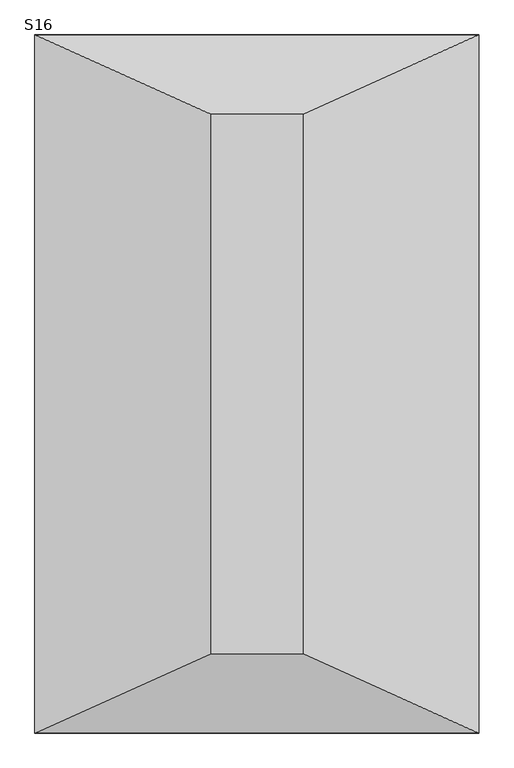
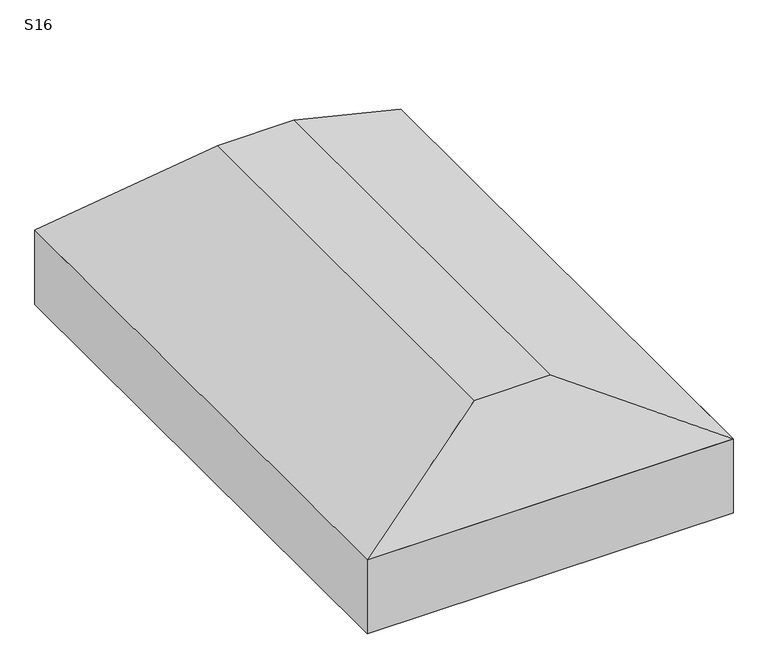
"""IFC4 building model written with IfcOpenShell, lengths in millimetres: fastener geometry, TQS - Sapata : S16."""

import ifcopenshell
import ifcopenshell.guid

model = None  # the IFC model being written
_history = None  # IfcOwnerHistory: only IFC2X3 demands one
_inside = {}  # id of a spatial element -> (the spatial element, [elements in it])
_under = {}  # id of a project, library or spatial element -> (it, [spatial elements below it])
_declared = {}  # id of a project -> (the project, [libraries it declares])
_typed = {}  # id of a type object -> (the type object, [elements of that type])
_made_of = {}  # id of a material, layer set ... -> (it, [elements and type objects made of it])


def new_model(schema):
    """Start an empty IFC model of exactly this schema.

    Asked for "IFC4X3", IfcOpenShell would pick the latest addendum, in which some entities
    have other attributes; the version numbers below select the first issue.
    IFC2X3 requires an IfcOwnerHistory on every rooted entity: one is made here for all.
    """
    global model, _history
    if schema == "IFC4X3":
        model = ifcopenshell.file(schema_version=(4, 3, 0, 0))
    else:
        model = ifcopenshell.file(schema=schema)
    _inside.clear()
    _under.clear()
    _declared.clear()
    _typed.clear()
    _made_of.clear()
    _history = None
    if model.schema == "IFC2X3":
        org = make("IfcOrganization", Name="unknown")
        user = make(
            "IfcPersonAndOrganization",
            ThePerson=make("IfcPerson", FamilyName="unknown"),
            TheOrganization=org,
        )
        app = make(
            "IfcApplication",
            ApplicationDeveloper=org,
            Version="unknown",
            ApplicationFullName="unknown",
            ApplicationIdentifier="unknown",
        )
        _history = make(
            "IfcOwnerHistory",
            OwningUser=user,
            OwningApplication=app,
            ChangeAction="ADDED",
            CreationDate=0,
        )
    return model


def make(cls, **values):
    """One entity of the class cls with the attributes given. An attribute that is None is left unset."""
    return model.create_entity(
        cls, **{name: value for name, value in values.items() if value is not None}
    )


def rooted(cls, **values):
    """An entity with a GlobalId (a new one), such as an element, a storey or a relation."""
    return make(cls, GlobalId=ifcopenshell.guid.new(), OwnerHistory=_history, **values)


def si_unit(unit_type, name, prefix=None):
    """IfcSIUnit, for example si_unit("LENGTHUNIT", "METRE", prefix="MILLI")."""
    return make("IfcSIUnit", UnitType=unit_type, Prefix=prefix, Name=name)


def assignment(units):
    """IfcUnitAssignment: the units of a project."""
    return None if units is None else make("IfcUnitAssignment", Units=units)


def point(xyz):
    """IfcCartesianPoint."""
    return None if xyz is None else make("IfcCartesianPoint", Coordinates=xyz)


def direction(xyz):
    """IfcDirection."""
    return None if xyz is None else make("IfcDirection", DirectionRatios=xyz)


def frame(location, z_axis=None, x_axis=None):
    """IfcAxis2Placement3D, a coordinate frame: its origin and axes. An axis left out is left unset."""
    return make(
        "IfcAxis2Placement3D",
        Location=point(location),
        Axis=direction(z_axis),
        RefDirection=direction(x_axis),
    )


def origin():
    """The frame at (0, 0, 0) with its axes left unset."""
    return frame((0.0, 0.0, 0.0))


def place(relative_to, where):
    """IfcLocalPlacement: puts the frame where relative to a parent placement (None: the world)."""
    return make(
        "IfcLocalPlacement", PlacementRelTo=relative_to, RelativePlacement=where
    )


def context(
    kind, dimensions, precision=None, world=None, true_north=None, identifier=None
):
    """IfcGeometricRepresentationContext, for example the 3D "Model" context."""
    return make(
        "IfcGeometricRepresentationContext",
        ContextIdentifier=identifier,
        ContextType=kind,
        CoordinateSpaceDimension=dimensions,
        Precision=precision,
        WorldCoordinateSystem=world,
        TrueNorth=true_north,
    )


def project(units=None, contexts=None):
    """IfcProject with its units and contexts."""
    return rooted(
        "IfcProject",
        Name="project",
        RepresentationContexts=contexts,
        UnitsInContext=assignment(units),
    )


def spatial(cls, under=None, at=None, **own):
    """A site, building, storey or space (cls), placed at a placement, below another one or the project."""
    s = rooted(cls, ObjectPlacement=at, **own)
    if under is not None:
        _under.setdefault(under.id(), (under, []))[1].append(s)
    return s


def polyline(points):
    """IfcPolyline through the points."""
    return make("IfcPolyline", Points=[point(p) for p in points])


def outline(outer, holes=None, kind="AREA"):
    """IfcArbitraryClosedProfileDef: a profile drawn as a closed curve; with holes, ...WithVoids."""
    if holes is None:
        return make("IfcArbitraryClosedProfileDef", ProfileType=kind, OuterCurve=outer)
    return make(
        "IfcArbitraryProfileDefWithVoids",
        ProfileType=kind,
        OuterCurve=outer,
        InnerCurves=holes,
    )


def extrude(swept, where, along, depth):
    """IfcExtrudedAreaSolid: the profile swept, set in the frame where, extruded along a direction by depth."""
    return make(
        "IfcExtrudedAreaSolid",
        SweptArea=swept,
        Position=where,
        ExtrudedDirection=direction(along),
        Depth=depth,
    )


def faces_of(points, faces, orient=None, outer=None):
    """IfcFace entities. A face is a list of loops; a loop is a list of indices into points, from 0.

    orient and outer hold one flag for each loop. By default every Orientation is true, the
    first loop of a face is its IfcFaceOuterBound and the others are IfcFaceBound.
    """
    made = []
    for i, loops in enumerate(faces):
        bounds = []
        for j, loop in enumerate(loops):
            is_outer = j == 0 if outer is None else outer[i][j]
            bounds.append(
                make(
                    "IfcFaceOuterBound" if is_outer else "IfcFaceBound",
                    Bound=make("IfcPolyLoop", Polygon=[points[k] for k in loop]),
                    Orientation=True if orient is None else orient[i][j],
                )
            )
        made.append(make("IfcFace", Bounds=bounds))
    return made


def faceted_brep(points, faces, orient=None, outer=None, voids=None):
    """IfcFacetedBrep: a solid bounded by flat faces; with voids (closed shells), ...WithVoids."""
    shared = [point(p) for p in points]
    hull = make("IfcClosedShell", CfsFaces=faces_of(shared, faces, orient, outer))
    if voids is None:
        return make("IfcFacetedBrep", Outer=hull)
    return make(
        "IfcFacetedBrepWithVoids",
        Outer=hull,
        Voids=[
            make(cls, CfsFaces=faces_of(shared, fs, o, b)) for cls, fs, o, b in voids
        ],
    )


def shape(context_of_items, identifier, shape_type, items):
    """IfcShapeRepresentation: the items that make up one representation, for example the "Body"."""
    return make(
        "IfcShapeRepresentation",
        ContextOfItems=context_of_items,
        RepresentationIdentifier=identifier,
        RepresentationType=shape_type,
        Items=items,
    )


def source(mapping_origin, context_of_items, identifier, shape_type, items):
    """IfcRepresentationMap: a shape defined once, which mapped items show again and again."""
    return make(
        "IfcRepresentationMap",
        MappingOrigin=mapping_origin,
        MappedRepresentation=shape(context_of_items, identifier, shape_type, items),
    )


def transform(
    local_origin,
    x_axis=None,
    y_axis=None,
    z_axis=None,
    scale=None,
    scale2=None,
    scale3=None,
    uniform=True,
):
    """IfcCartesianTransformationOperator3D, or its non-uniform kind. x_axis, y_axis, z_axis: its Axis1, 2, 3."""
    if uniform:
        return make(
            "IfcCartesianTransformationOperator3D",
            Axis1=direction(x_axis),
            Axis2=direction(y_axis),
            LocalOrigin=point(local_origin),
            Scale=scale,
            Axis3=direction(z_axis),
        )
    return make(
        "IfcCartesianTransformationOperator3DnonUniform",
        Axis1=direction(x_axis),
        Axis2=direction(y_axis),
        LocalOrigin=point(local_origin),
        Scale=scale,
        Axis3=direction(z_axis),
        Scale2=scale2,
        Scale3=scale3,
    )


def mapped(mapping_source, mapping_target):
    """IfcMappedItem: shows the shape of a source again, moved by a transform."""
    return make(
        "IfcMappedItem", MappingSource=mapping_source, MappingTarget=mapping_target
    )


def made_of(thing, what):
    """Note that an element or type object is made of a material, layer set ...; save() writes the relation."""
    if what is not None:
        _made_of.setdefault(what.id(), (what, []))[1].append(thing)
    return thing


def element(
    cls,
    number,
    at=None,
    inside=None,
    cuts=None,
    type_object=None,
    material=None,
    context=None,
    identifier="Body",
    shape_type=None,
    held_by="IfcProductDefinitionShape",
    body=None,
    shapes=None,
    **own,
):
    """One element of the class cls, such as IfcWall. Its Tag is "e" and its number.

    at: its placement. inside: the storey or other place that contains it. cuts: it is an
    opening in that element (IfcRelVoidsElement). A single representation is given by context,
    identifier, shape_type and body (its items); several are given by shapes. held_by: the class
    of the entity that holds the representations. save() writes the other relations.
    """
    e = rooted(cls, Tag="e%d" % number, ObjectPlacement=at, **own)
    if body is not None:
        shapes = [shape(context, identifier, shape_type, body)]
    if shapes is not None:
        e.Representation = make(held_by, Representations=shapes)
    if inside is not None:
        _inside.setdefault(inside.id(), (inside, []))[1].append(e)
    if cuts is not None:
        rooted(
            "IfcRelVoidsElement", RelatingBuildingElement=cuts, RelatedOpeningElement=e
        )
    if type_object is not None:
        _typed.setdefault(type_object.id(), (type_object, []))[1].append(e)
    return made_of(e, material)


def aggregate(whole, parts):
    """IfcRelAggregates: a whole, such as a stair, and the parts it consists of."""
    return rooted("IfcRelAggregates", RelatingObject=whole, RelatedObjects=parts)


def save(model, path):
    """Write the relations noted so far, then the file.

    IfcRelAggregates (storeys below a building ...), IfcRelContainedInSpatialStructure (elements
    in a storey), IfcRelDefinesByType, IfcRelAssociatesMaterial and IfcRelDeclares: one each for
    every whole, place, type object, material and project.
    """
    for whole, parts in _under.values():
        aggregate(whole, parts)
    for where, things in _inside.values():
        rooted(
            "IfcRelContainedInSpatialStructure",
            RelatedElements=things,
            RelatingStructure=where,
        )
    for kind, things in _typed.values():
        rooted("IfcRelDefinesByType", RelatedObjects=things, RelatingType=kind)
    for what, things in _made_of.values():
        rooted("IfcRelAssociatesMaterial", RelatedObjects=things, RelatingMaterial=what)
    for by, libraries in _declared.values():
        rooted("IfcRelDeclares", RelatingContext=by, RelatedDefinitions=libraries)
    model.write(path)


def s16_25b1d231(model_context):
    return source(origin(), model_context, "Body", "SolidModel", [
        faceted_brep([(-55.0, 650.0, 0.0), (-345.0, 650.0, 0.0), (-345.0, -1050.0, 0.0), (-55.0, -1050.0, 0.0), (500.0, 900.0, -300.0), (500.0, -1300.0, -300.0), (-900.0, -1300.0, -300.0), (-900.0, 900.0, -300.0)], [[[0, 1, 2, 3]], [[4, 5, 6, 7]], [[4, 7, 1, 0]], [[7, 6, 2, 1]], [[6, 5, 3, 2]], [[5, 4, 0, 3]]]),
        extrude(outline(polyline([(500.0, 900.0), (500.0, -1300.0), (-900.0, -1300.0), (-900.0, 900.0), (500.0, 900.0)])), frame((0.0, 0.0, -600.0), z_axis=(0.0, 0.0, 1.0), x_axis=(1.0, 0.0, 0.0)), (0.0, 0.0, 1.0), 300.0),
    ])


if __name__ == "__main__":
    model = new_model("IFC4")
    model_context = context("Model", 3, world=origin())
    ifc_project = project(units=[si_unit("LENGTHUNIT", "METRE", prefix="MILLI")], contexts=[model_context])
    site = spatial("IfcSite", under=ifc_project)
    building = spatial("IfcBuilding", under=site)
    placement = place(None, origin())
    s16_shape = s16_25b1d231(model_context)
    element("IfcFastener", 1, ObjectType="TQS - Sapata : S16", at=placement, inside=building, context=model_context, shape_type="MappedRepresentation", body=[
        mapped(s16_shape, transform((0.0, 0.0, 0.0), x_axis=(1.0, 0.0, 0.0), y_axis=(0.0, 1.0, 0.0), z_axis=(0.0, 0.0, 1.0))),
    ])
    save(model, "model.ifc")

# Revit data of these elements
# Type "TQS - Sapata : S16"
#   TY = 1.70 m
#   TX = 0.29 m
#   HS = 0.60 m
#   H0 = 0.30 m
#   EXCYABS = 1.10 m
#   EXCY = 0.00 m
#   EXCXABS = 0.70 m
#   EXCX = 0.00 m
#   DIMY = 2.20 m
#   DIMX = 1.40 m
#   Material estrutural = Concreto - Concreto concretado no local
#   Width = 0
#   Length = 0
# Element 1 (IfcFastener, "TQS - Sapata : S16")
#   Materials on its faces: "Concreto - Concreto concretado no local"
# Materials
#   "Concreto - Concreto concretado no local": class "Concreto", colour RGB 192 192 192, transparency 0
